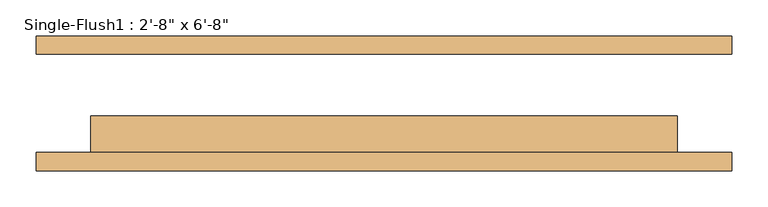
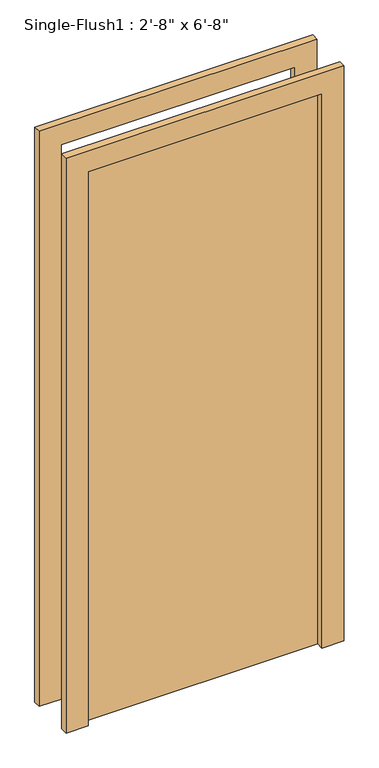
"""IFC4 building model written with IfcOpenShell, lengths in millimetres: door geometry."""

from ifc_helpers import new_model, si_unit, frame, origin, origin_with_axes, place, context, project, spatial, polyline, outline, extrude, source, transform, mapped, element, save


def door_a239bf7e(model_context):
    return source(origin(), model_context, "Body", "SweptSolid", [
        extrude(outline(polyline([(2108.2, -482.6), (0.0, -482.6), (0.0, -406.4), (2032.0, -406.4), (2032.0, 406.4), (0.0, 406.4), (0.0, 482.6), (2108.2, 482.6), (2108.2, -482.6)])), frame((0.0, -93.6625, 0.0), z_axis=(0.0, 1.0, 0.0), x_axis=(0.0, 0.0, 1.0)), (0.0, 0.0, 1.0), 25.4),
        extrude(outline(polyline([(2108.2, 482.6), (2108.2, -482.6), (0.0, -482.6), (0.0, -406.4), (2032.0, -406.4), (2032.0, 406.4), (0.0, 406.4), (0.0, 482.6), (2108.2, 482.6)])), frame((0.0, 68.2625, 0.0), z_axis=(0.0, 1.0, 0.0), x_axis=(0.0, 0.0, 1.0)), (0.0, 0.0, 1.0), 25.4),
        extrude(outline(polyline([(406.4, -17.4625), (406.4, -68.2625), (-406.4, -68.2625), (-406.4, -17.4625), (406.4, -17.4625)])), origin_with_axes(), (0.0, 0.0, 1.0), 2032.0),
    ])


if __name__ == "__main__":
    model = new_model("IFC4")
    model_context = context("Model", 3, world=origin())
    ifc_project = project(units=[si_unit("LENGTHUNIT", "METRE", prefix="MILLI")], contexts=[model_context])
    site = spatial("IfcSite", under=ifc_project)
    building = spatial("IfcBuilding", under=site)
    placement = place(None, origin())
    door_shape = door_a239bf7e(model_context)
    element("IfcDoor", 1, ObjectType="Single-Flush1 : 2'-8\" x 6'-8\"", at=placement, inside=building, context=model_context, shape_type="MappedRepresentation", body=[
        mapped(door_shape, transform((0.0, 0.0, 0.0), x_axis=(1.0, 0.0, 0.0), y_axis=(0.0, 1.0, 0.0), z_axis=(0.0, 0.0, 1.0))),
    ])
    save(model, "model.ifc")

# Revit data of these elements
# Type "Single-Flush1 : 2'-8\" x 6'-8\""
#   Type Mark = "D4"
#   Construction Type Id = "MDOOR"
#   Assembly Code = "C1020"
#   Analytic Construction = "Metal"
#   Thickness = 0' - 2"
#   Heat Transfer Coefficient (U) = 3.7021 W/(m²·K)
#   Height = 6' - 8"
#   Trim Projection Ext = 0' - 1"
#   Trim Projection Int = 0' - 1"
#   Trim Width = 0' - 3"
#   Width = 2' - 8"
#   Door Material = Door - Panel
#   Frame Material = Door - Frame
#   Visual Light Transmittance = 0
#   Solar Heat Gain Coefficient = 0
#   Function = (empty or 0)
#   Wall Closure = (empty or 0)
# Element 1 (IfcDoor, "Single-Flush1 : 2'-8\" x 6'-8\"")
#   Materials on its faces: "Door - Frame", "Door - Panel"
# Materials
#   "Door - Panel": class "Wood", colour RGB 210 159 95, transparency 0, Cost = 0
#   "Door - Frame": class "Miscellaneous", colour RGB 118 70 51, transparency 0, Cost = 0
